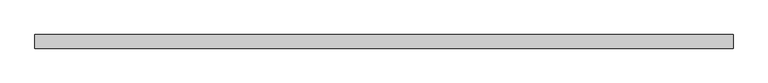
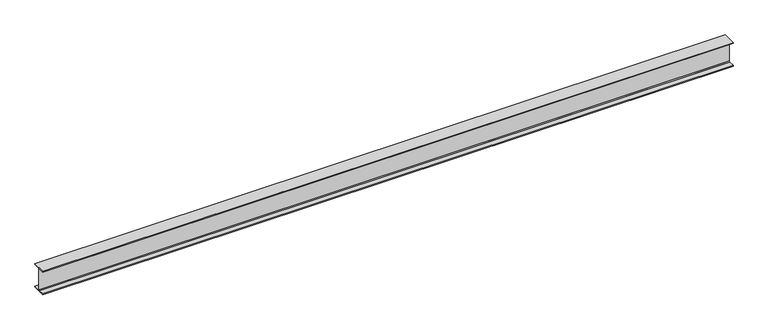
"""IFC4 building model written with IfcOpenShell, lengths in millimetres: beam geometry, Old_Steel Beam_H-KSD3502 : H_SB_ASB_H-800×300x14x26."""

from ifc_helpers import new_model, si_unit, point, frame, frame_2d, origin, place, context, project, spatial, polyline, circle_curve, trimmed, segment, composite_curve, outline, extrude, source, transform, mapped, element, save


def beam_f6b0f30e(model_context):
    return source(origin(), model_context, "Body", "SweptSolid", [
        extrude(outline(composite_curve([segment(polyline([(82.5, -141.5), (82.5, -151.7), (-82.5, -151.7), (-82.5, -141.5), (-11.9, -141.5)]), True, "CONTINUOUS"), segment(trimmed(circle_curve(frame_2d((-11.9, -132.6)), 8.9), [point((-11.9, -141.5))], [point((-3.0, -132.6))], True, "CARTESIAN"), True, "CONTINUOUS"), segment(polyline([(-3.0, -132.6), (-3.0, 132.6)]), True, "CONTINUOUS"), segment(trimmed(circle_curve(frame_2d((-11.9, 132.6)), 8.9), [point((-3.0, 132.6))], [point((-11.9, 141.5))], True, "CARTESIAN"), True, "CONTINUOUS"), segment(polyline([(-11.9, 141.5), (-82.5, 141.5), (-82.5, 151.7), (82.5, 151.7), (82.5, 141.5), (11.9, 141.5)]), True, "CONTINUOUS"), segment(trimmed(circle_curve(frame_2d((11.9, 132.6)), 8.9), [point((11.9, 141.5))], [point((3.0, 132.6))], True, "CARTESIAN"), True, "CONTINUOUS"), segment(polyline([(3.0, 132.6), (3.0, -132.6)]), True, "CONTINUOUS"), segment(trimmed(circle_curve(frame_2d((11.9, -132.6)), 8.9), [point((3.0, -132.6))], [point((11.9, -141.5))], True, "CARTESIAN"), True, "CONTINUOUS"), segment(polyline([(11.9, -141.5), (82.5, -141.5)]), True, "CONTINUOUS")], self_intersect=False)), frame((-4285.8606617, 0.0, 0.0), z_axis=(1.0, 0.0, 0.0), x_axis=(0.0, 1.0, 0.0)), (0.0, 0.0, 1.0), 8443.8590445),
    ])


if __name__ == "__main__":
    model = new_model("IFC4")
    model_context = context("Model", 3, world=origin())
    ifc_project = project(units=[si_unit("LENGTHUNIT", "METRE", prefix="MILLI")], contexts=[model_context])
    site = spatial("IfcSite", under=ifc_project)
    building = spatial("IfcBuilding", under=site)
    placement = place(None, origin())
    beam_shape = beam_f6b0f30e(model_context)
    element("IfcBeam", 1, ObjectType="Old_Steel Beam_H-KSD3502 : H_SB_ASB_H-800×300x14x26", at=placement, inside=building, context=model_context, shape_type="MappedRepresentation", body=[
        mapped(beam_shape, transform((0.0, 0.0, 0.0), x_axis=(1.0, 0.0, 0.0), y_axis=(0.0, 1.0, 0.0), z_axis=(0.0, 0.0, 1.0))),
    ])
    save(model, "model.ifc")

# Revit data of these elements
# Type "Old_Steel Beam_H-KSD3502 : H_SB_ASB_H-800×300x14x26"
#   Width = 30.0 cm
#   Web Thickness = 1.4 cm
#   Web Fillet = 2.8 cm
#   Warping Constant = 17523000.0 cm⁶
#   Torsional Moment of Inertia = 422.315 cm⁴
#   Torsional Modulus = 1.0 cm³
#   Section Area = 267.4 cm²
#   Plastic Modulus weak axis = 1220.0 cm³
#   Plastic Modulus strong axis = 8240.0 cm³
#   Perimeter = 2.72 m²/m
#   Nominal Weight = 210.00 kgf/m
#   Moment of Inertia weak axis = 11700.00 cm⁴
#   Moment of Inertia strong axis = 292000.00 cm⁴
#   Height = 80.0 cm
#   Flange Thickness = 2.6 cm
#   Elastic Modulus weak axis = 782.0 cm³
#   Elastic Modulus strong axis = 7290.0 cm³
#   Centroid Vertical = 40.0 cm
#   Centroid Horizontal = 15.0 cm
#   Length [instance default] = 1.5240 m
#   Structural Material [instance default] = Steel, 45-345
#   Assembly Code = ""
# Element 1 (IfcBeam, "Old_Steel Beam_H-KSD3502 : H_SB_ASB_H-800×300x14x26")
#   Structural Material = none
# Materials
#   "Steel, 45-345": class "Metal", colour RGB 189 187 185, transparency 0, Description = "Steel 345 MPa", Cost = 0
